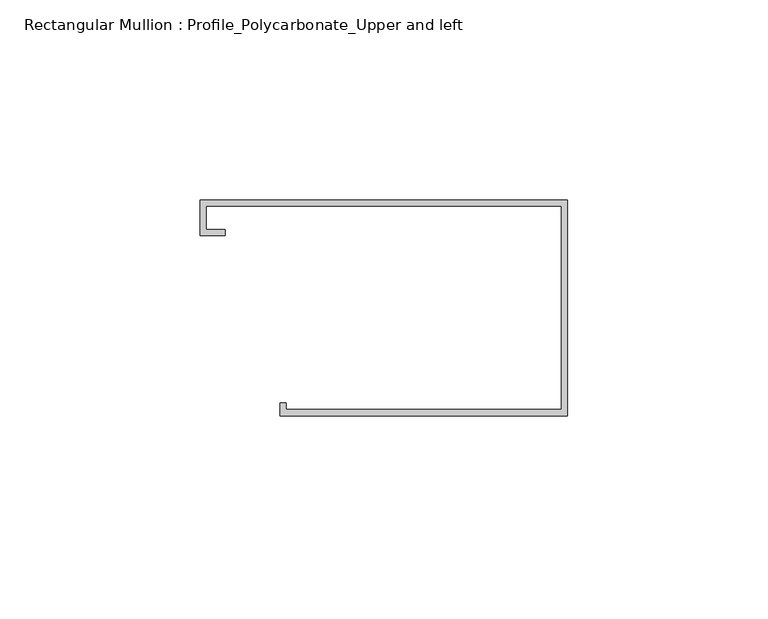
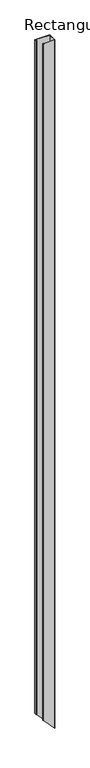
"""IFC4 building model written with IfcOpenShell, lengths in millimetres: member geometry, Rectangular Mullion : Profile_Polycarbonate_Upper and left."""

from ifc_helpers import new_model, si_unit, origin, place, context, project, spatial, faceted_brep, source, transform, mapped, element, save


def rectangular_mullion_profile_polycarbonate_upper_and_left_79227f0d(model_context):
    return source(origin(), model_context, "Body", "Brep", [
        faceted_brep([(0.0, 28.984575, 0.0), (-91.9988, 28.984575, 0.0), (-91.9988, 19.992975, 0.0), (-85.6488, 19.992975, 0.0), (-85.6488, 21.580475, 0.0), (-90.4113, 21.580475, 0.0), (-90.4113, 27.397075, 0.0), (-1.5875, 27.397075, 0.0), (-1.5875, -23.428325, 0.0), (-70.3961, -23.428325, 0.0), (-70.3961, -21.840825, 0.0), (-71.9836, -21.840825, 0.0), (-71.9836, -25.015825, 0.0), (0.0, -25.015825, 0.0), (0.0, 28.984575, -4472.3181431), (-91.9988, 28.984575, -4376.4062343), (-91.9988, 19.992975, -4376.4062343), (-85.6488, 19.992975, -4383.0263274), (-85.6488, 21.580475, -4383.0263274), (-90.4113, 21.580475, -4378.0612576), (-90.4113, 27.397075, -4378.0612576), (-1.5875, 27.397075, -4470.6631198), (-1.5875, -23.428325, -4470.6631198), (-70.3961, -23.428325, -4398.9277911), (-70.3961, -21.840825, -4398.9277911), (-71.9836, -21.840825, -4397.2727678), (-71.9836, -25.015825, -4397.2727678), (0.0, -25.015825, -4472.3181431)], [[[0, 1, 2, 3, 4, 5, 6, 7, 8, 9, 10, 11, 12, 13]], [[1, 0, 14, 15]], [[2, 1, 15, 16]], [[3, 2, 16, 17]], [[4, 3, 17, 18]], [[5, 4, 18, 19]], [[6, 5, 19, 20]], [[7, 6, 20, 21]], [[8, 7, 21, 22]], [[9, 8, 22, 23]], [[10, 9, 23, 24]], [[11, 10, 24, 25]], [[12, 11, 25, 26]], [[13, 12, 26, 27]], [[0, 13, 27, 14]], [[14, 27, 26, 25, 24, 23, 22, 21, 20, 19, 18, 17, 16, 15]]]),
    ])


if __name__ == "__main__":
    model = new_model("IFC4")
    model_context = context("Model", 3, world=origin())
    ifc_project = project(units=[si_unit("LENGTHUNIT", "METRE", prefix="MILLI")], contexts=[model_context])
    site = spatial("IfcSite", under=ifc_project)
    building = spatial("IfcBuilding", under=site)
    placement = place(None, origin())
    rectangular_mullion_profile_polycarbonate_upper_and_left_shape = rectangular_mullion_profile_polycarbonate_upper_and_left_79227f0d(model_context)
    element("IfcMember", 1, ObjectType="Rectangular Mullion : Profile_Polycarbonate_Upper and left", at=placement, inside=building, context=model_context, shape_type="MappedRepresentation", body=[
        mapped(rectangular_mullion_profile_polycarbonate_upper_and_left_shape, transform((0.0, 0.0, 0.0), x_axis=(1.0, 0.0, 0.0), y_axis=(0.0, 1.0, 0.0), z_axis=(0.0, 0.0, 1.0))),
    ])
    save(model, "model.ifc")

# Revit data of these elements
# Type "Rectangular Mullion : Profile_Polycarbonate_Upper and left"
#   built-in parameter 1007322 = 0.177167 (stored number, unit not read)
#   built-in parameter 1007321 = 0.00520833 (stored number, unit not read)
#   built-in parameter 1007320 = 0 (stored number, unit not read)
